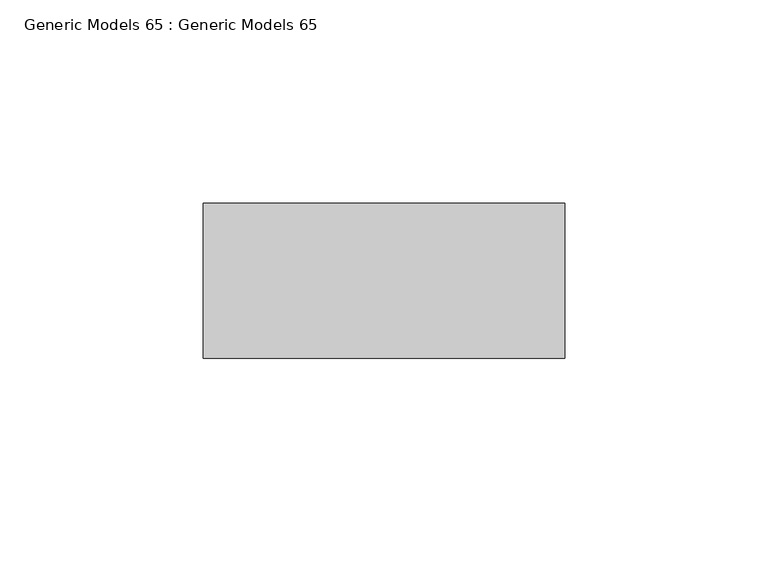
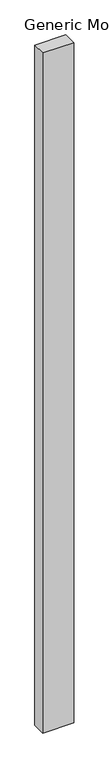
"""IFC4 building model written with IfcOpenShell, lengths in millimetres: proxy geometry, Generic Models 65 : Generic Models 65."""

from ifc_helpers import new_model, si_unit, frame, origin, place, context, project, spatial, polyline, outline, extrude, source, transform, mapped, element, save


def generic_models_65_generic_models_65_eaa428f0(model_context):
    return source(origin(), model_context, "Body", "SweptSolid", [
        extrude(outline(polyline([(51003.2, 592.1375), (50914.3, 592.1375), (50914.3, 630.2375), (51003.2, 630.2375), (51003.2, 592.1375)])), frame((0.0, 0.0, 3086.1), z_axis=(0.0, 0.0, 1.0), x_axis=(1.0, 0.0, 0.0)), (0.0, 0.0, 1.0), 2060.178125),
    ])


if __name__ == "__main__":
    model = new_model("IFC4")
    model_context = context("Model", 3, world=origin())
    ifc_project = project(units=[si_unit("LENGTHUNIT", "METRE", prefix="MILLI")], contexts=[model_context])
    site = spatial("IfcSite", under=ifc_project)
    building = spatial("IfcBuilding", under=site)
    placement = place(None, origin())
    generic_models_65_generic_models_65_shape = generic_models_65_generic_models_65_eaa428f0(model_context)
    element("IfcBuildingElementProxy", 1, Name="Generic Models 65 : Generic Models 65", ObjectType="Generic Models 65 : Generic Models 65", at=placement, inside=building, context=model_context, shape_type="MappedRepresentation", body=[
        mapped(generic_models_65_generic_models_65_shape, transform((0.0, 0.0, 0.0), x_axis=(1.0, 0.0, 0.0), y_axis=(0.0, 1.0, 0.0), z_axis=(0.0, 0.0, 1.0))),
    ])
    save(model, "model.ifc")

# Revit data of these elements
# Element 1 (IfcBuildingElementProxy, "Generic Models 65 : Generic Models 65")
#   Materials on its faces: "2X WOOD STUD - SEE 'WALL TAG' & 'LAYER MATERIAL SCHEDULE' FOR SPACING & INSULATION TREATMENT, IF APPLICAPLE"
# Materials
#   "2X WOOD STUD - SEE 'WALL TAG' & 'LAYER MATERIAL SCHEDULE' FOR SPACING & INSULATION TREATMENT, IF APPLICAPLE": class "Wood", colour RGB 234 198 147, transparency 0, Description = "Pinus Echinata", Cost = 0
